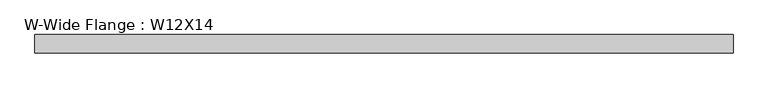
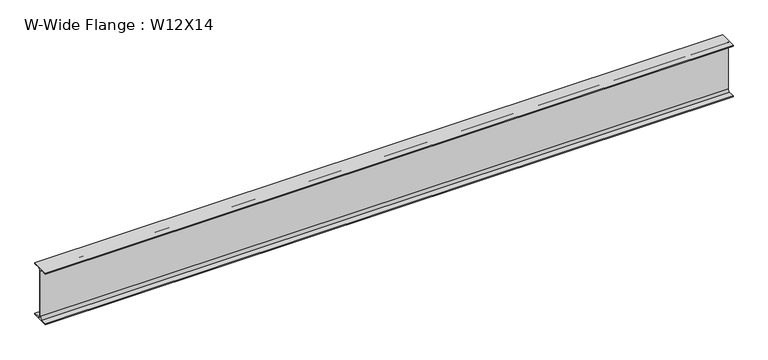
"""IFC4 building model written with IfcOpenShell, lengths in millimetres: beam geometry, W-Wide Flange : W12X14."""

from ifc_helpers import new_model, si_unit, point, frame, frame_2d, origin, place, context, project, spatial, polyline, circle_curve, trimmed, segment, composite_curve, outline, extrude, source, transform, mapped, element, save


def w_wide_flange_w12x14_02e3ecd4(model_context):
    return source(origin(), model_context, "Body", "SweptSolid", [
        extrude(outline(composite_curve([segment(polyline([(50.419, -145.415), (50.419, -151.13), (-50.419, -151.13), (-50.419, -145.415), (-15.875, -145.415)]), True, "CONTINUOUS"), segment(trimmed(circle_curve(frame_2d((-15.875, -132.08)), 13.335), [point((-15.875, -145.415))], [point((-2.54, -132.08))], True, "CARTESIAN"), True, "CONTINUOUS"), segment(polyline([(-2.54, -132.08), (-2.54, 132.08)]), True, "CONTINUOUS"), segment(trimmed(circle_curve(frame_2d((-15.875, 132.08)), 13.335), [point((-2.54, 132.08))], [point((-15.875, 145.415))], True, "CARTESIAN"), True, "CONTINUOUS"), segment(polyline([(-15.875, 145.415), (-50.419, 145.415), (-50.419, 151.13), (50.419, 151.13), (50.419, 145.415), (15.875, 145.415)]), True, "CONTINUOUS"), segment(trimmed(circle_curve(frame_2d((15.875, 132.08)), 13.335), [point((15.875, 145.415))], [point((2.54, 132.08))], True, "CARTESIAN"), True, "CONTINUOUS"), segment(polyline([(2.54, 132.08), (2.54, -132.08)]), True, "CONTINUOUS"), segment(trimmed(circle_curve(frame_2d((15.875, -132.08)), 13.335), [point((2.54, -132.08))], [point((15.875, -145.415))], True, "CARTESIAN"), True, "CONTINUOUS"), segment(polyline([(15.875, -145.415), (50.419, -145.415)]), True, "CONTINUOUS")], self_intersect=False)), frame((-1905.0, 0.0, 0.0), z_axis=(1.0, 0.0, 0.0), x_axis=(0.0, 1.0, 0.0)), (0.0, 0.0, 1.0), 3810.0),
    ])


if __name__ == "__main__":
    model = new_model("IFC4")
    model_context = context("Model", 3, world=origin())
    ifc_project = project(units=[si_unit("LENGTHUNIT", "METRE", prefix="MILLI")], contexts=[model_context])
    site = spatial("IfcSite", under=ifc_project)
    building = spatial("IfcBuilding", under=site)
    placement = place(None, origin())
    w_wide_flange_w12x14_shape = w_wide_flange_w12x14_02e3ecd4(model_context)
    element("IfcBeam", 1, ObjectType="W-Wide Flange : W12X14", at=placement, inside=building, context=model_context, shape_type="MappedRepresentation", body=[
        mapped(w_wide_flange_w12x14_shape, transform((0.0, 0.0, 0.0), x_axis=(1.0, 0.0, 0.0), y_axis=(0.0, 1.0, 0.0), z_axis=(0.0, 0.0, 1.0))),
    ])
    save(model, "model.ifc")

# Revit data of these elements
# Type "W-Wide Flange : W12X14"
#   Assembly Code = "B10"
#   W = 14
#   Length [instance default] = 5' - 0"
#   bf = 0' - 3.97"
#   d = 0' - 11.9"
#   k = 0' - 0 3/4"
#   k2 = 0' - 0.525"
#   tf = 0' - 0.225"
#   tw = 0' - 0.2"
#   A = 0.0288889 SF
#   Structural Material [instance default] = Steel ASTM A992
# Element 1 (IfcBeam, "W-Wide Flange : W12X14")
#   Materials on its faces: "Steel ASTM A992"
# Materials
#   "Steel ASTM A992": class "Metal", colour RGB 199 199 199, transparency 0, Description = "Structural steel 50ksi", Cost = 0
